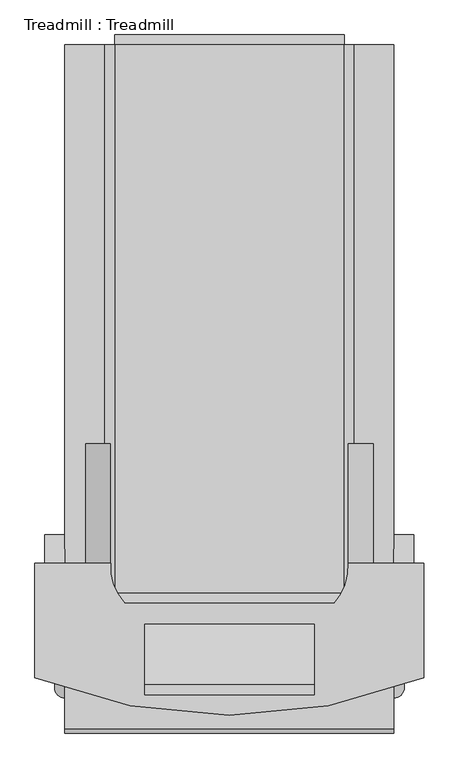
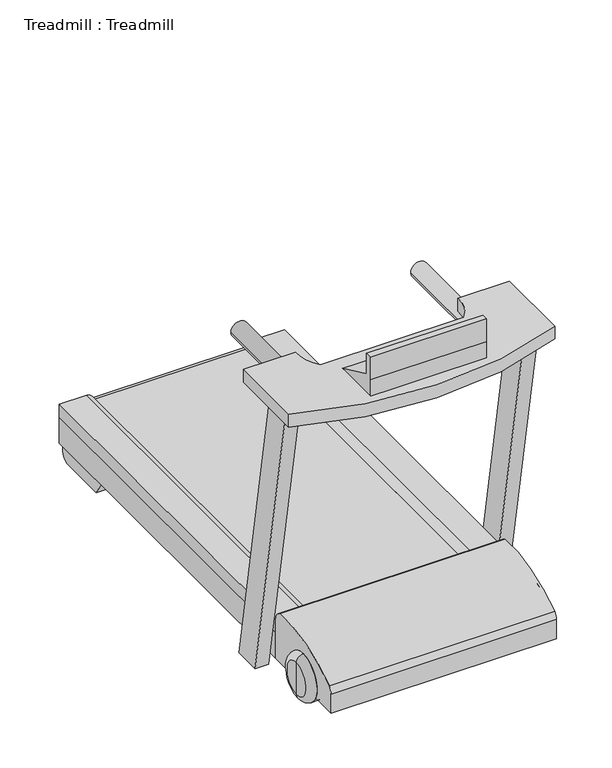
"""IFC4 building model written with IfcOpenShell, lengths in millimetres: proxy geometry, Treadmill : Treadmill."""

from ifc_helpers import new_model, si_unit, point, frame, frame_2d, origin, place, context, project, spatial, polyline, circle_curve, ellipse_curve, trimmed, segment, composite_curve, outline, extrude, source, transform, mapped, element, save
from ifc_brep_helpers import plane_surface, cylinder_surface, revolved_surface, advanced_brep


def treadmill_treadmill_2e70c73b(model_context):
    return source(origin(), model_context, "Body", "SolidModel", [
        advanced_brep(
        [(838.2, 177.8, 88.9), (838.2, 177.8, 0.0), (838.2, 177.8, 177.8), (889.7314789, 177.8, 151.7399805), (889.7314789, 177.8, 26.0600195), (889.7314789, 177.8, 88.9), (863.6714594, 177.8, 177.8), (863.6714594, 177.8, 0.0)],
        [
            (0, 1),
            (1, 2, circle_curve(frame((838.2, 177.8, 88.9), z_axis=(-1.0, 0.0, 0.0), x_axis=(0.0, 0.0, -1.0)), 88.9)),
            (2, 0),
            (2, 1, circle_curve(frame((838.2, 177.8, 88.9), z_axis=(-1.0, 0.0, 0.0), x_axis=(0.0, 0.0, -1.0)), 88.9)),
            (3, 4, circle_curve(frame((889.7314789, 177.8, 88.9), z_axis=(1.0, 0.0, 0.0), x_axis=(0.0, 0.0, -1.0)), 62.8399805)),
            (4, 5),
            (5, 3),
            (4, 3, circle_curve(frame((889.7314789, 177.8, 88.9), z_axis=(1.0, 0.0, 0.0), x_axis=(0.0, 0.0, -1.0)), 62.8399805)),
            (6, 7, circle_curve(frame((863.6714594, 177.8, 88.9), z_axis=(1.0, 0.0, 0.0), x_axis=(0.0, 0.0, -1.0)), 88.9)),
            (7, 4, circle_curve(frame((863.6714594, 177.8, 26.0600195), z_axis=(0.0, -1.0, 0.0), x_axis=(0.0, 0.0, -1.0)), 26.0600195)),
            (3, 6, circle_curve(frame((863.6714594, 177.8, 151.7399805), z_axis=(0.0, -1.0, 0.0), x_axis=(0.0, 0.0, 1.0)), 26.0600195)),
            (7, 6, circle_curve(frame((863.6714594, 177.8, 88.9), z_axis=(1.0, 0.0, 0.0), x_axis=(0.0, 0.0, -1.0)), 88.9)),
            (1, 7),
            (6, 2),
        ],
        [
            plane_surface(frame((838.2, 177.8, 88.9), z_axis=(-1.0, 0.0, 0.0), x_axis=(0.0, 0.0, -1.0))),
            plane_surface(frame((889.7314789, 177.8, 88.9), z_axis=(1.0, 0.0, 0.0), x_axis=(0.0, 0.0, -1.0))),
            revolved_surface(trimmed(ellipse_curve(frame((863.6714594, 177.8, 26.0600195), z_axis=(0.0, 1.0, 0.0), x_axis=(0.0, 0.0, -1.0)), 26.0600195, 26.0600195), [point((889.7314789, 177.8, 26.0600195))], [point((863.6714594, 177.8, 0.0))], True, "CARTESIAN"), (889.7314789, 177.8, 88.9), (-1.0, 0.0, 0.0)),
            cylinder_surface(frame((889.7314789, 177.8, 88.9), z_axis=(-1.0, 0.0, 0.0), x_axis=(0.0, 0.0, -1.0)), 88.9),
        ],
        [
            (0, [[1, 2, 3]]),
            (0, [[-3, 4, -1]]),
            (1, [[5, 6, 7]]),
            (1, [[8, -7, -6]]),
            (2, [[9, 10, -5, 11]]),
            (2, [[12, -11, -8, -10]]),
            (3, [[-2, 13, -9, 14]]),
            (3, [[-4, -14, -12, -13]]),
        ],
    ),
        advanced_brep(
        [(25.3285406, 177.8, 177.8), (25.3285406, 177.8, 0.0), (50.8, 177.8, 0.0), (50.8, 177.8, 177.8), (-0.7314789, 177.8, 151.7399805), (-0.7314789, 177.8, 26.0600195), (-0.7314789, 177.8, 88.9), (50.8, 177.8, 88.9)],
        [
            (0, 1, circle_curve(frame((25.3285406, 177.8, 88.9), z_axis=(1.0, 0.0, 0.0), x_axis=(0.0, 0.0, -1.0)), 88.9)),
            (1, 2),
            (2, 3, circle_curve(frame((50.8, 177.8, 88.9), z_axis=(-1.0, 0.0, 0.0), x_axis=(0.0, 0.0, -1.0)), 88.9)),
            (3, 0),
            (1, 0, circle_curve(frame((25.3285406, 177.8, 88.9), z_axis=(1.0, 0.0, 0.0), x_axis=(0.0, 0.0, -1.0)), 88.9)),
            (3, 2, circle_curve(frame((50.8, 177.8, 88.9), z_axis=(-1.0, 0.0, 0.0), x_axis=(0.0, 0.0, -1.0)), 88.9)),
            (4, 5, circle_curve(frame((-0.7314789, 177.8, 88.9), z_axis=(1.0, 0.0, 0.0), x_axis=(0.0, 0.0, -1.0)), 62.8399805)),
            (5, 1, circle_curve(frame((25.3285406, 177.8, 26.0600195), z_axis=(0.0, -1.0, 0.0), x_axis=(0.0, 0.0, -1.0)), 26.0600195)),
            (0, 4, circle_curve(frame((25.3285406, 177.8, 151.7399805), z_axis=(0.0, -1.0, 0.0), x_axis=(0.0, 0.0, 1.0)), 26.0600195)),
            (5, 4, circle_curve(frame((-0.7314789, 177.8, 88.9), z_axis=(1.0, 0.0, 0.0), x_axis=(0.0, 0.0, -1.0)), 62.8399805)),
            (6, 5),
            (4, 6),
            (2, 7),
            (7, 3),
        ],
        [
            cylinder_surface(frame((-0.7314789, 177.8, 88.9), z_axis=(-1.0, 0.0, 0.0), x_axis=(0.0, 0.0, -1.0)), 88.9),
            revolved_surface(trimmed(ellipse_curve(frame((25.3285406, 177.8, 26.0600195), z_axis=(0.0, 1.0, 0.0), x_axis=(0.0, 0.0, -1.0)), 26.0600195, 26.0600195), [point((25.3285406, 177.8, 0.0))], [point((-0.7314789, 177.8, 26.0600195))], True, "CARTESIAN"), (-0.7314789, 177.8, 88.9), (-1.0, 0.0, 0.0)),
            plane_surface(frame((-0.7314789, 177.8, 88.9), z_axis=(-1.0, 0.0, 0.0), x_axis=(0.0, 0.0, -1.0))),
            plane_surface(frame((50.8, 177.8, 88.9), z_axis=(1.0, 0.0, 0.0), x_axis=(0.0, 0.0, -1.0))),
        ],
        [
            (0, [[1, 2, 3, 4]]),
            (0, [[5, -4, 6, -2]]),
            (1, [[7, 8, -1, 9]]),
            (1, [[10, -9, -5, -8]]),
            (2, [[11, -7, 12]]),
            (2, [[-12, -10, -11]]),
            (3, [[-3, 13, 14]]),
            (3, [[-6, -14, -13]]),
        ],
    ),
        extrude(outline(composite_curve([segment(polyline([(355.6, 152.4), (355.6, 177.8), (1752.6, 177.8)]), True, "CONTINUOUS"), segment(trimmed(circle_curve(frame_2d((1752.6, 152.4)), 25.4), [point((1752.6, 177.8))], [point((1752.6, 127.0))], False, "CARTESIAN"), True, "CONTINUOUS"), segment(polyline([(1752.6, 127.0), (1752.6, 152.4), (355.6, 152.4)]), True, "CONTINUOUS")], self_intersect=False)), frame((152.4, 0.0, 0.0), z_axis=(1.0, 0.0, 0.0), x_axis=(0.0, 1.0, 0.0)), (0.0, 0.0, 1.0), 584.2),
        extrude(outline(composite_curve([segment(polyline([(356.6198638, 50.8), (0.0, 50.8), (0.0, 127.0)]), True, "CONTINUOUS"), segment(trimmed(circle_curve(frame_2d((36.1581881, 127.0)), 36.1581881), [point((0.0, 127.0))], [point((10.4238809, 152.4))], False, "CARTESIAN"), True, "CONTINUOUS"), segment(trimmed(circle_curve(frame_2d((289.1455701, -230.6771793)), 473.744557), [point((10.4238809, 152.4))], [point((330.6373426, 241.2469016))], False, "CARTESIAN"), True, "CONTINUOUS"), segment(trimmed(circle_curve(frame_2d((319.002006, 205.4588927)), 37.6319364), [point((330.6373426, 241.2469016))], [point((356.6198638, 204.4296136))], False, "CARTESIAN"), True, "CONTINUOUS"), segment(polyline([(356.6198638, 204.4296136), (356.6198638, 50.8)]), True, "CONTINUOUS")], self_intersect=False)), frame((25.4, 0.0, 0.0), z_axis=(1.0, 0.0, 0.0), x_axis=(0.0, 1.0, 0.0)), (0.0, 0.0, 1.0), 838.2),
        extrude(outline(composite_curve([segment(polyline([(152.4, 152.4), (177.8, 152.4)]), True, "CONTINUOUS"), segment(trimmed(circle_curve(frame_2d((177.8, 127.0)), 25.4), [point((177.8, 152.4))], [point((203.2, 127.0))], False, "CARTESIAN"), True, "CONTINUOUS"), segment(polyline([(203.2, 127.0), (203.2, 25.4), (152.4, 25.4), (50.8, 25.4), (50.8, 863.6), (152.4, 863.6), (203.2, 863.6), (203.2, 762.0)]), True, "CONTINUOUS"), segment(trimmed(circle_curve(frame_2d((177.8, 762.0)), 25.4), [point((203.2, 762.0))], [point((177.8, 736.6))], False, "CARTESIAN"), True, "CONTINUOUS"), segment(polyline([(177.8, 736.6), (152.4, 736.6), (152.4, 152.4)]), True, "CONTINUOUS")], self_intersect=False)), frame((0.0, 355.6, 0.0), z_axis=(0.0, 1.0, 0.0), x_axis=(0.0, 0.0, 1.0)), (0.0, 0.0, 1.0), 1397.0),
        extrude(outline(polyline([(122.6746955, 1240.8350591), (277.1099218, 1168.4), (97.2746955, 1168.4), (97.2746955, 1231.9), (97.2746955, 1320.8), (122.6746955, 1320.8), (122.6746955, 1240.8350591)])), frame((228.6, 0.0, 0.0), z_axis=(1.0, 0.0, 0.0), x_axis=(0.0, 1.0, 0.0)), (0.0, 0.0, 1.0), 431.8),
        advanced_brep(
        [(78.1863004, 736.6, 1085.0214532), (141.6863004, 736.6, 1085.0214532), (78.1863004, 229.0227686, 1085.0214532), (141.6863004, 255.3253298, 1085.0214532), (128.3884153, 178.8206537, 1085.0214532), (154.6909766, 242.3206537, 1085.0214532), (760.6115847, 178.8206537, 1085.0214532), (734.3090234, 242.3206537, 1085.0214532), (810.8136996, 229.0227686, 1085.0214532), (747.3136996, 255.3253298, 1085.0214532), (810.8136996, 736.6, 1085.0214532), (747.3136996, 736.6, 1085.0214532)],
        [
            (0, 1, circle_curve(frame((109.9363004, 736.6, 1085.0214532), z_axis=(0.0, 1.0, 0.0), x_axis=(1.0, 0.0, 0.0)), 31.75)),
            (1, 0, circle_curve(frame((109.9363004, 736.6, 1085.0214532), z_axis=(0.0, 1.0, 0.0), x_axis=(1.0, 0.0, 0.0)), 31.75)),
            (0, 2),
            (2, 3, ellipse_curve(frame((109.9363004, 242.1740492, 1085.0214532), z_axis=(-0.382683432365089, 0.9238795325112871, 0.0), x_axis=(0.9238795325112872, 0.3826834323650889, 0.0)), 34.3659524, 31.75)),
            (3, 1),
            (3, 2, ellipse_curve(frame((109.9363004, 242.1740492, 1085.0214532), z_axis=(-0.382683432365089, 0.9238795325112871, 0.0), x_axis=(0.9238795325112872, 0.3826834323650889, 0.0)), 34.3659524, 31.75)),
            (2, 4),
            (4, 5, ellipse_curve(frame((141.5396959, 210.5706537, 1085.0214532), z_axis=(-0.9238795325112865, 0.3826834323650906, 0.0), x_axis=(0.38268343236509084, 0.9238795325112864, 0.0)), 34.3659524, 31.75)),
            (5, 3),
            (5, 4, ellipse_curve(frame((141.5396959, 210.5706537, 1085.0214532), z_axis=(-0.9238795325112865, 0.3826834323650906, 0.0), x_axis=(0.38268343236509084, 0.9238795325112864, 0.0)), 34.3659524, 31.75)),
            (4, 6),
            (6, 7, ellipse_curve(frame((747.4603041, 210.5706537, 1085.0214532), z_axis=(-0.9238795325112865, -0.3826834323650905, 0.0), x_axis=(-0.38268343236509034, 0.9238795325112866, 0.0)), 34.3659524, 31.75)),
            (7, 5),
            (7, 6, ellipse_curve(frame((747.4603041, 210.5706537, 1085.0214532), z_axis=(-0.9238795325112865, -0.3826834323650905, 0.0), x_axis=(-0.38268343236509034, 0.9238795325112866, 0.0)), 34.3659524, 31.75)),
            (6, 8),
            (8, 9, ellipse_curve(frame((779.0636996, 242.1740492, 1085.0214532), z_axis=(-0.382683432365089, -0.923879532511287, 0.0), x_axis=(-0.9238795325112873, 0.38268343236508884, 0.0)), 34.3659524, 31.75)),
            (9, 7),
            (9, 8, ellipse_curve(frame((779.0636996, 242.1740492, 1085.0214532), z_axis=(-0.382683432365089, -0.923879532511287, 0.0), x_axis=(-0.9238795325112873, 0.38268343236508884, 0.0)), 34.3659524, 31.75)),
            (10, 11, circle_curve(frame((779.0636996, 736.6, 1085.0214532), z_axis=(0.0, 1.0, 0.0), x_axis=(-1.0, 0.0, 0.0)), 31.75)),
            (11, 10, circle_curve(frame((779.0636996, 736.6, 1085.0214532), z_axis=(0.0, 1.0, 0.0), x_axis=(-1.0, 0.0, 0.0)), 31.75)),
            (8, 10),
            (11, 9),
        ],
        [
            plane_surface(frame((-1038.8645002, 736.6, 0.0), z_axis=(0.0, 1.0, 0.0), x_axis=(0.0, 0.0, -1.0))),
            cylinder_surface(frame((109.9363004, 736.6, 1085.0214532), z_axis=(0.0, 1.0, 0.0), x_axis=(1.0, 0.0, 0.0)), 31.75),
            cylinder_surface(frame((100.3379982, 251.7723515, 1085.0214532), z_axis=(-0.7071067811865464, 0.7071067811865488, 0.0), x_axis=(0.7071067811865488, 0.7071067811865464, 0.0)), 31.75),
            cylinder_surface(frame((127.9656467, 210.5706537, 1085.0214532), z_axis=(-1.0, 0.0, 0.0), x_axis=(0.0, 1.0, 0.0)), 31.75),
            cylinder_surface(frame((737.8620018, 200.9723515, 1085.0214532), z_axis=(-0.7071067811865465, -0.7071067811865487, 0.0), x_axis=(-0.7071067811865487, 0.7071067811865465, 0.0)), 31.75),
            plane_surface(frame((-304.1957937, 736.6, 0.0), z_axis=(0.0, 1.0, 0.0), x_axis=(0.0, 0.0, 1.0))),
            cylinder_surface(frame((779.0636996, 228.6, 1085.0214532), z_axis=(0.0, -1.0, 0.0), x_axis=(-1.0, 0.0, 0.0)), 31.75),
        ],
        [
            (0, [[1, 2]]),
            (1, [[-1, 3, 4, 5]]),
            (1, [[-2, -5, 6, -3]]),
            (2, [[-4, 7, 8, 9]]),
            (2, [[-6, -9, 10, -7]]),
            (3, [[-8, 11, 12, 13]]),
            (3, [[-10, -13, 14, -11]]),
            (4, [[-12, 15, 16, 17]]),
            (4, [[-14, -17, 18, -15]]),
            (5, [[19, 20]]),
            (6, [[-16, 21, -20, 22]]),
            (6, [[-18, -22, -19, -21]]),
        ],
    ),
        extrude(outline(composite_curve([segment(polyline([(-50.8, 141.347801), (-50.8, 432.8198638), (142.1724844, 432.8198638)]), True, "CONTINUOUS"), segment(trimmed(circle_curve(frame_2d((276.1196867, 422.2461786)), 134.3638933), [point((142.1724844, 432.8198638))], [point((177.8268743, 330.6373426))], True, "CARTESIAN"), True, "CONTINUOUS"), segment(polyline([(177.8268743, 330.6373426), (711.1731257, 330.6373426)]), True, "CONTINUOUS"), segment(trimmed(circle_curve(frame_2d((612.8803133, 422.2461786)), 134.3638933), [point((711.1731257, 330.6373426))], [point((746.8275156, 432.8198638))], True, "CARTESIAN"), True, "CONTINUOUS"), segment(polyline([(746.8275156, 432.8198638), (939.8, 432.8198638), (939.8, 141.347801)]), True, "CONTINUOUS"), segment(trimmed(circle_curve(frame_2d((444.5, 1366.4086936)), 1321.3993645), [point((939.8, 141.347801))], [point((-50.8, 141.347801))], False, "CARTESIAN"), True, "CONTINUOUS")], self_intersect=False)), frame((0.0, 0.0, 1117.6), z_axis=(0.0, 0.0, 1.0), x_axis=(1.0, 0.0, 0.0)), (0.0, 0.0, 1.0), 50.8),
        extrude(outline(polyline([(204.732057, 1117.6), (307.8994008, 1117.6), (504.9624344, 0.0), (401.7950906, 0.0), (204.732057, 1117.6)])), frame((-25.4, 0.0, 0.0), z_axis=(1.0, 0.0, 0.0), x_axis=(0.0, 1.0, 0.0)), (0.0, 0.0, 1.0), 50.8),
        extrude(outline(polyline([(204.732057, 1117.6), (307.8994008, 1117.6), (504.9624344, 0.0), (401.7950906, 0.0), (204.732057, 1117.6)])), frame((863.6, 0.0, 0.0), z_axis=(1.0, 0.0, 0.0), x_axis=(0.0, 1.0, 0.0)), (0.0, 0.0, 1.0), 50.8),
        extrude(outline(composite_curve([segment(polyline([(1514.6655035, 0.0), (1483.7010673, 50.8), (1731.2449893, 50.8), (1731.2449893, 38.1)]), True, "CONTINUOUS"), segment(trimmed(circle_curve(frame_2d((1693.1449893, 38.1)), 38.1), [point((1731.2449893, 38.1))], [point((1693.1449893, 0.0))], False, "CARTESIAN"), True, "CONTINUOUS"), segment(polyline([(1693.1449893, 0.0), (1514.6655035, 0.0)]), True, "CONTINUOUS")], self_intersect=False)), frame((25.4, 0.0, 0.0), z_axis=(1.0, 0.0, 0.0), x_axis=(0.0, 1.0, 0.0)), (0.0, 0.0, 1.0), 838.2),
    ])


if __name__ == "__main__":
    model = new_model("IFC4")
    model_context = context("Model", 3, world=origin())
    ifc_project = project(units=[si_unit("LENGTHUNIT", "METRE", prefix="MILLI")], contexts=[model_context])
    site = spatial("IfcSite", under=ifc_project)
    building = spatial("IfcBuilding", under=site)
    placement = place(None, origin())
    treadmill_treadmill_shape = treadmill_treadmill_2e70c73b(model_context)
    element("IfcBuildingElementProxy", 1, Name="Treadmill : Treadmill", ObjectType="Treadmill : Treadmill", at=placement, inside=building, context=model_context, shape_type="MappedRepresentation", body=[
        mapped(treadmill_treadmill_shape, transform((0.0, 0.0, 0.0), x_axis=(1.0, 0.0, 0.0), y_axis=(0.0, 1.0, 0.0), z_axis=(0.0, 0.0, 1.0))),
    ])
    save(model, "model.ifc")

# Revit data of these elements
# Type "Treadmill : Treadmill"
#   Keynote = "N"
#   Assembly Code = "E1090"
# Element 1 (IfcBuildingElementProxy, "Treadmill : Treadmill")
#   Materials on its faces: "Metal - Steel", "Pastic - Black"
# Materials
#   "Metal - Steel": class "Unassigned", colour RGB 247 247 247, transparency 0
#   "Pastic - Black": class "Unassigned", colour RGB 255 255 255, transparency 0, Cost = 0
